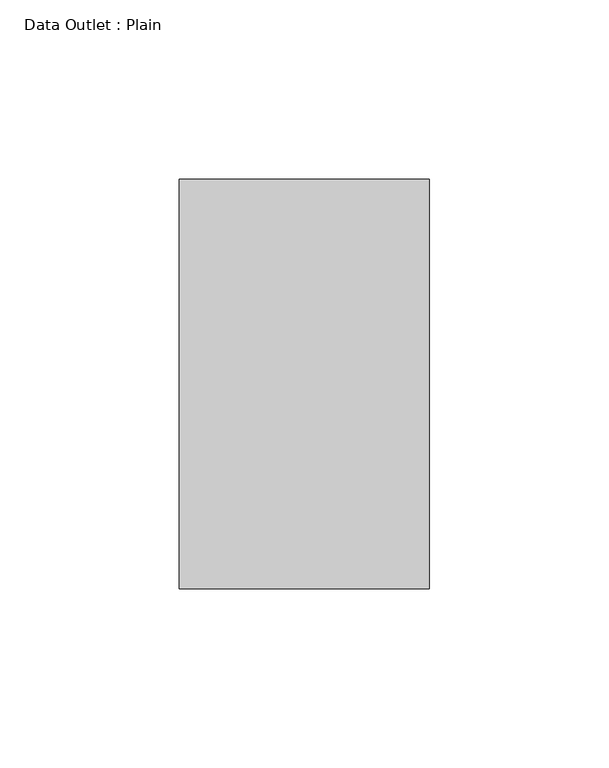
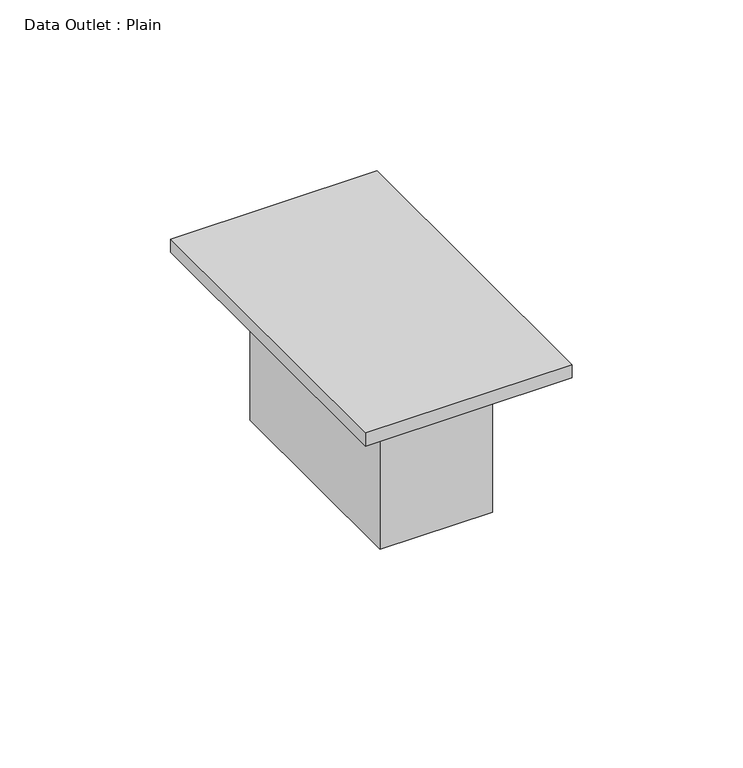
"""IFC4 building model written with IfcOpenShell, lengths in millimetres: electric appliance geometry, Data Outlet : Plain."""

from ifc_helpers import new_model, si_unit, frame, origin, origin_with_axes, place, context, project, spatial, polyline, outline, extrude, source, transform, mapped, element, save


def data_outlet_plain_367a9a66(model_context):
    return source(origin(), model_context, "Body", "SweptSolid", [
        extrude(outline(polyline([(34.925, 57.15), (34.925, -57.15), (-34.925, -57.15), (-34.925, 57.15), (34.925, 57.15)])), origin_with_axes(), (0.0, 0.0, 1.0), 4.7625),
        extrude(outline(polyline([(19.05, 38.1), (19.05, -38.1), (-19.05, -38.1), (-19.05, 38.1), (19.05, 38.1)])), frame((0.0, 0.0, -53.975), z_axis=(0.0, 0.0, 1.0), x_axis=(1.0, 0.0, 0.0)), (0.0, 0.0, 1.0), 53.975),
    ])


if __name__ == "__main__":
    model = new_model("IFC4")
    model_context = context("Model", 3, world=origin())
    ifc_project = project(units=[si_unit("LENGTHUNIT", "METRE", prefix="MILLI")], contexts=[model_context])
    site = spatial("IfcSite", under=ifc_project)
    building = spatial("IfcBuilding", under=site)
    placement = place(None, origin())
    data_outlet_plain_shape = data_outlet_plain_367a9a66(model_context)
    element("IfcElectricAppliance", 1, ObjectType="Data Outlet : Plain", at=placement, inside=building, context=model_context, shape_type="MappedRepresentation", body=[
        mapped(data_outlet_plain_shape, transform((0.0, 0.0, 0.0), x_axis=(1.0, 0.0, 0.0), y_axis=(0.0, 1.0, 0.0), z_axis=(0.0, 0.0, 1.0))),
    ])
    save(model, "model.ifc")

# Revit data of these elements
# Type "Data Outlet : Plain"
#   Label = ""
#   Default Elevation = 1' - 6"
#   Assembly Code = ""
